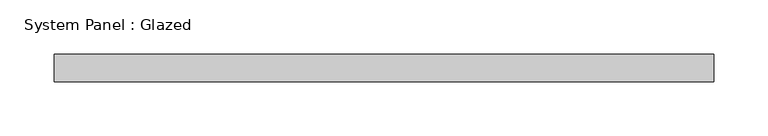
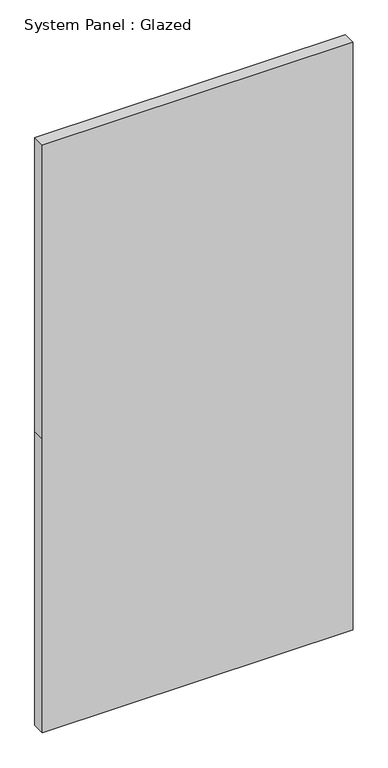
"""IFC4 building model written with IfcOpenShell, lengths in millimetres: plate geometry, System Panel : Glazed."""

from ifc_helpers import new_model, si_unit, frame, origin, place, context, project, spatial, polyline, outline, extrude, source, transform, mapped, element, save


def system_panel_glazed_b14f9832(model_context):
    return source(origin(), model_context, "Body", "SweptSolid", [
        extrude(outline(polyline([(0.0, -304.8), (0.0, 304.8), (609.6, 304.8), (1219.2, 304.8), (1219.2, -304.8), (609.6, -304.8), (0.0, -304.8)])), frame((0.0, 19.05, 0.0), z_axis=(0.0, 1.0, 0.0), x_axis=(0.0, 0.0, 1.0)), (0.0, 0.0, 1.0), 25.4),
    ])


if __name__ == "__main__":
    model = new_model("IFC4")
    model_context = context("Model", 3, world=origin())
    ifc_project = project(units=[si_unit("LENGTHUNIT", "METRE", prefix="MILLI")], contexts=[model_context])
    site = spatial("IfcSite", under=ifc_project)
    building = spatial("IfcBuilding", under=site)
    placement = place(None, origin())
    system_panel_glazed_shape = system_panel_glazed_b14f9832(model_context)
    element("IfcPlate", 1, ObjectType="System Panel : Glazed", at=placement, inside=building, context=model_context, shape_type="MappedRepresentation", body=[
        mapped(system_panel_glazed_shape, transform((0.0, 0.0, 0.0), x_axis=(1.0, 0.0, 0.0), y_axis=(0.0, 1.0, 0.0), z_axis=(0.0, 0.0, 1.0))),
    ])
    save(model, "model.ifc")

# Revit data of these elements
# Element 1 (IfcPlate, "System Panel : Glazed")
#   Materials on its faces: "Glass"
# Materials
#   "Glass": class "Glass", colour RGB 0 128 192, transparency 0.75
